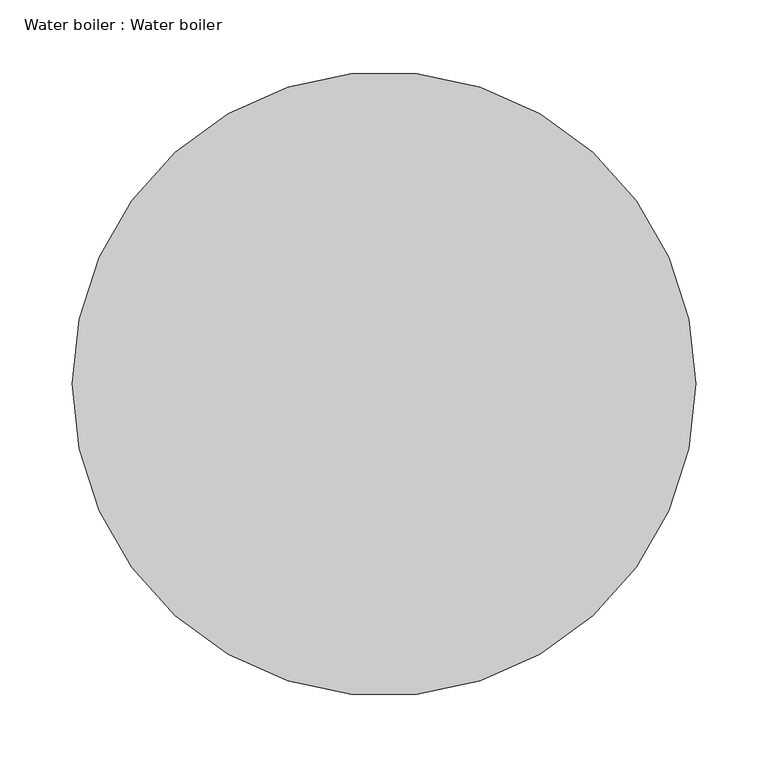
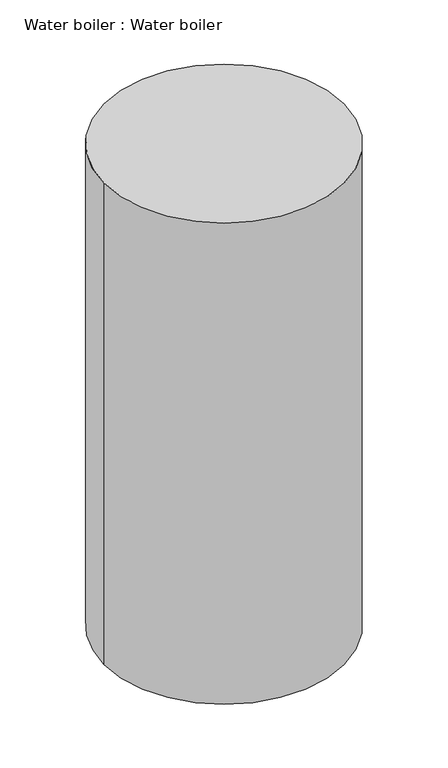
"""IFC4 building model written with IfcOpenShell, lengths in millimetres: proxy geometry, Water boiler : Water boiler."""

from ifc_helpers import new_model, si_unit, point, frame, frame_2d, origin, place, context, project, spatial, circle_curve, trimmed, segment, composite_curve, outline, extrude, source, transform, mapped, element, save


def water_boiler_water_boiler_54bea4d4(model_context):
    return source(origin(), model_context, "Body", "SweptSolid", [
        extrude(outline(composite_curve([segment(trimmed(circle_curve(frame_2d((25724.6370052, 10998.0325125)), 215.9), [point((25508.7370052, 10998.0325125))], [point((25940.5370052, 10998.0325125))], False, "CARTESIAN"), True, "CONTINUOUS"), segment(trimmed(circle_curve(frame_2d((25724.6370052, 10998.0325125)), 215.9), [point((25940.5370052, 10998.0325125))], [point((25508.7370052, 10998.0325125))], False, "CARTESIAN"), True, "CONTINUOUS")], self_intersect=False)), frame((0.0, 0.0, 2832.1), z_axis=(0.0, 0.0, 1.0), x_axis=(1.0, 0.0, 0.0)), (0.0, 0.0, 1.0), 914.4),
    ])


if __name__ == "__main__":
    model = new_model("IFC4")
    model_context = context("Model", 3, world=origin())
    ifc_project = project(units=[si_unit("LENGTHUNIT", "METRE", prefix="MILLI")], contexts=[model_context])
    site = spatial("IfcSite", under=ifc_project)
    building = spatial("IfcBuilding", under=site)
    placement = place(None, origin())
    water_boiler_water_boiler_shape = water_boiler_water_boiler_54bea4d4(model_context)
    element("IfcBuildingElementProxy", 1, Name="Water boiler : Water boiler", ObjectType="Water boiler : Water boiler", at=placement, inside=building, context=model_context, shape_type="MappedRepresentation", body=[
        mapped(water_boiler_water_boiler_shape, transform((0.0, 0.0, 0.0), x_axis=(1.0, 0.0, 0.0), y_axis=(0.0, 1.0, 0.0), z_axis=(0.0, 0.0, 1.0))),
    ])
    save(model, "model.ifc")
